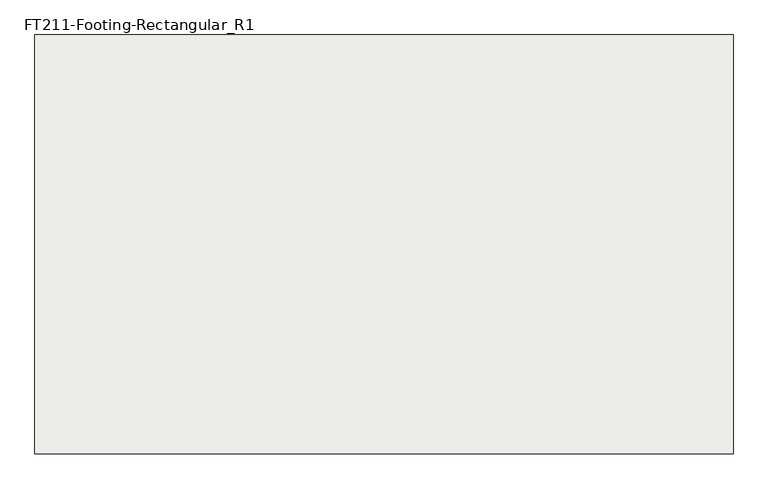
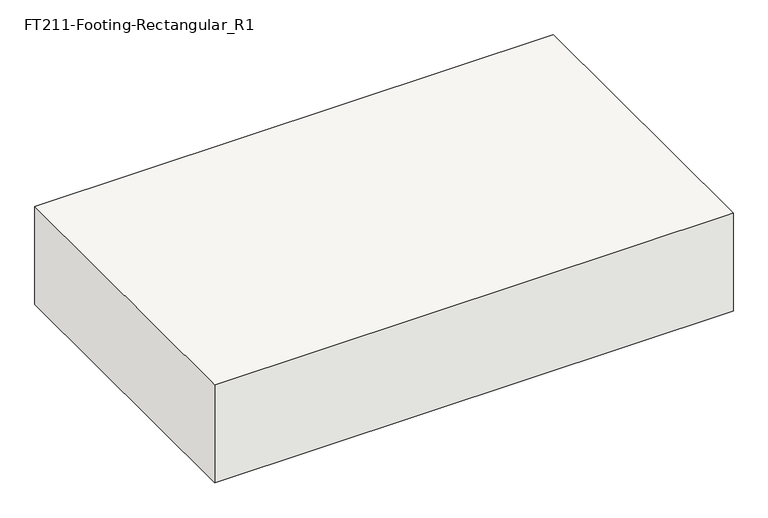
"""IFC4 building model written with IfcOpenShell, lengths in millimetres: slab geometry, FT211-Footing-Rectangular_R1 : H_SF_ACF_W2500xL1500xT500_Bitumen."""

import ifcopenshell
import ifcopenshell.guid

model = None  # the IFC model being written
_history = None  # IfcOwnerHistory: only IFC2X3 demands one
_inside = {}  # id of a spatial element -> (the spatial element, [elements in it])
_under = {}  # id of a project, library or spatial element -> (it, [spatial elements below it])
_declared = {}  # id of a project -> (the project, [libraries it declares])
_typed = {}  # id of a type object -> (the type object, [elements of that type])
_made_of = {}  # id of a material, layer set ... -> (it, [elements and type objects made of it])


def new_model(schema):
    """Start an empty IFC model of exactly this schema.

    Asked for "IFC4X3", IfcOpenShell would pick the latest addendum, in which some entities
    have other attributes; the version numbers below select the first issue.
    IFC2X3 requires an IfcOwnerHistory on every rooted entity: one is made here for all.
    """
    global model, _history
    if schema == "IFC4X3":
        model = ifcopenshell.file(schema_version=(4, 3, 0, 0))
    else:
        model = ifcopenshell.file(schema=schema)
    _inside.clear()
    _under.clear()
    _declared.clear()
    _typed.clear()
    _made_of.clear()
    _history = None
    if model.schema == "IFC2X3":
        org = make("IfcOrganization", Name="unknown")
        user = make(
            "IfcPersonAndOrganization",
            ThePerson=make("IfcPerson", FamilyName="unknown"),
            TheOrganization=org,
        )
        app = make(
            "IfcApplication",
            ApplicationDeveloper=org,
            Version="unknown",
            ApplicationFullName="unknown",
            ApplicationIdentifier="unknown",
        )
        _history = make(
            "IfcOwnerHistory",
            OwningUser=user,
            OwningApplication=app,
            ChangeAction="ADDED",
            CreationDate=0,
        )
    return model


def make(cls, **values):
    """One entity of the class cls with the attributes given. An attribute that is None is left unset."""
    return model.create_entity(
        cls, **{name: value for name, value in values.items() if value is not None}
    )


def rooted(cls, **values):
    """An entity with a GlobalId (a new one), such as an element, a storey or a relation."""
    return make(cls, GlobalId=ifcopenshell.guid.new(), OwnerHistory=_history, **values)


def si_unit(unit_type, name, prefix=None):
    """IfcSIUnit, for example si_unit("LENGTHUNIT", "METRE", prefix="MILLI")."""
    return make("IfcSIUnit", UnitType=unit_type, Prefix=prefix, Name=name)


def assignment(units):
    """IfcUnitAssignment: the units of a project."""
    return None if units is None else make("IfcUnitAssignment", Units=units)


def point(xyz):
    """IfcCartesianPoint."""
    return None if xyz is None else make("IfcCartesianPoint", Coordinates=xyz)


def direction(xyz):
    """IfcDirection."""
    return None if xyz is None else make("IfcDirection", DirectionRatios=xyz)


def frame(location, z_axis=None, x_axis=None):
    """IfcAxis2Placement3D, a coordinate frame: its origin and axes. An axis left out is left unset."""
    return make(
        "IfcAxis2Placement3D",
        Location=point(location),
        Axis=direction(z_axis),
        RefDirection=direction(x_axis),
    )


def origin():
    """The frame at (0, 0, 0) with its axes left unset."""
    return frame((0.0, 0.0, 0.0))


def place(relative_to, where):
    """IfcLocalPlacement: puts the frame where relative to a parent placement (None: the world)."""
    return make(
        "IfcLocalPlacement", PlacementRelTo=relative_to, RelativePlacement=where
    )


def context(
    kind, dimensions, precision=None, world=None, true_north=None, identifier=None
):
    """IfcGeometricRepresentationContext, for example the 3D "Model" context."""
    return make(
        "IfcGeometricRepresentationContext",
        ContextIdentifier=identifier,
        ContextType=kind,
        CoordinateSpaceDimension=dimensions,
        Precision=precision,
        WorldCoordinateSystem=world,
        TrueNorth=true_north,
    )


def project(units=None, contexts=None):
    """IfcProject with its units and contexts."""
    return rooted(
        "IfcProject",
        Name="project",
        RepresentationContexts=contexts,
        UnitsInContext=assignment(units),
    )


def spatial(cls, under=None, at=None, **own):
    """A site, building, storey or space (cls), placed at a placement, below another one or the project."""
    s = rooted(cls, ObjectPlacement=at, **own)
    if under is not None:
        _under.setdefault(under.id(), (under, []))[1].append(s)
    return s


def polyline(points):
    """IfcPolyline through the points."""
    return make("IfcPolyline", Points=[point(p) for p in points])


def outline(outer, holes=None, kind="AREA"):
    """IfcArbitraryClosedProfileDef: a profile drawn as a closed curve; with holes, ...WithVoids."""
    if holes is None:
        return make("IfcArbitraryClosedProfileDef", ProfileType=kind, OuterCurve=outer)
    return make(
        "IfcArbitraryProfileDefWithVoids",
        ProfileType=kind,
        OuterCurve=outer,
        InnerCurves=holes,
    )


def extrude(swept, where, along, depth):
    """IfcExtrudedAreaSolid: the profile swept, set in the frame where, extruded along a direction by depth."""
    return make(
        "IfcExtrudedAreaSolid",
        SweptArea=swept,
        Position=where,
        ExtrudedDirection=direction(along),
        Depth=depth,
    )


def shape(context_of_items, identifier, shape_type, items):
    """IfcShapeRepresentation: the items that make up one representation, for example the "Body"."""
    return make(
        "IfcShapeRepresentation",
        ContextOfItems=context_of_items,
        RepresentationIdentifier=identifier,
        RepresentationType=shape_type,
        Items=items,
    )


def source(mapping_origin, context_of_items, identifier, shape_type, items):
    """IfcRepresentationMap: a shape defined once, which mapped items show again and again."""
    return make(
        "IfcRepresentationMap",
        MappingOrigin=mapping_origin,
        MappedRepresentation=shape(context_of_items, identifier, shape_type, items),
    )


def transform(
    local_origin,
    x_axis=None,
    y_axis=None,
    z_axis=None,
    scale=None,
    scale2=None,
    scale3=None,
    uniform=True,
):
    """IfcCartesianTransformationOperator3D, or its non-uniform kind. x_axis, y_axis, z_axis: its Axis1, 2, 3."""
    if uniform:
        return make(
            "IfcCartesianTransformationOperator3D",
            Axis1=direction(x_axis),
            Axis2=direction(y_axis),
            LocalOrigin=point(local_origin),
            Scale=scale,
            Axis3=direction(z_axis),
        )
    return make(
        "IfcCartesianTransformationOperator3DnonUniform",
        Axis1=direction(x_axis),
        Axis2=direction(y_axis),
        LocalOrigin=point(local_origin),
        Scale=scale,
        Axis3=direction(z_axis),
        Scale2=scale2,
        Scale3=scale3,
    )


def mapped(mapping_source, mapping_target):
    """IfcMappedItem: shows the shape of a source again, moved by a transform."""
    return make(
        "IfcMappedItem", MappingSource=mapping_source, MappingTarget=mapping_target
    )


def made_of(thing, what):
    """Note that an element or type object is made of a material, layer set ...; save() writes the relation."""
    if what is not None:
        _made_of.setdefault(what.id(), (what, []))[1].append(thing)
    return thing


def element(
    cls,
    number,
    at=None,
    inside=None,
    cuts=None,
    type_object=None,
    material=None,
    context=None,
    identifier="Body",
    shape_type=None,
    held_by="IfcProductDefinitionShape",
    body=None,
    shapes=None,
    **own,
):
    """One element of the class cls, such as IfcWall. Its Tag is "e" and its number.

    at: its placement. inside: the storey or other place that contains it. cuts: it is an
    opening in that element (IfcRelVoidsElement). A single representation is given by context,
    identifier, shape_type and body (its items); several are given by shapes. held_by: the class
    of the entity that holds the representations. save() writes the other relations.
    """
    e = rooted(cls, Tag="e%d" % number, ObjectPlacement=at, **own)
    if body is not None:
        shapes = [shape(context, identifier, shape_type, body)]
    if shapes is not None:
        e.Representation = make(held_by, Representations=shapes)
    if inside is not None:
        _inside.setdefault(inside.id(), (inside, []))[1].append(e)
    if cuts is not None:
        rooted(
            "IfcRelVoidsElement", RelatingBuildingElement=cuts, RelatedOpeningElement=e
        )
    if type_object is not None:
        _typed.setdefault(type_object.id(), (type_object, []))[1].append(e)
    return made_of(e, material)


def aggregate(whole, parts):
    """IfcRelAggregates: a whole, such as a stair, and the parts it consists of."""
    return rooted("IfcRelAggregates", RelatingObject=whole, RelatedObjects=parts)


def save(model, path):
    """Write the relations noted so far, then the file.

    IfcRelAggregates (storeys below a building ...), IfcRelContainedInSpatialStructure (elements
    in a storey), IfcRelDefinesByType, IfcRelAssociatesMaterial and IfcRelDeclares: one each for
    every whole, place, type object, material and project.
    """
    for whole, parts in _under.values():
        aggregate(whole, parts)
    for where, things in _inside.values():
        rooted(
            "IfcRelContainedInSpatialStructure",
            RelatedElements=things,
            RelatingStructure=where,
        )
    for kind, things in _typed.values():
        rooted("IfcRelDefinesByType", RelatedObjects=things, RelatingType=kind)
    for what, things in _made_of.values():
        rooted("IfcRelAssociatesMaterial", RelatedObjects=things, RelatingMaterial=what)
    for by, libraries in _declared.values():
        rooted("IfcRelDeclares", RelatingContext=by, RelatedDefinitions=libraries)
    model.write(path)


def ft211_footing_rectangular_r1_907a7f09(model_context):
    return source(origin(), model_context, "Body", "SweptSolid", [
        extrude(outline(polyline([(1250.0, 750.0), (1250.0, -750.0), (-1250.0, -750.0), (-1250.0, 750.0), (1250.0, 750.0)])), frame((0.0, 0.0, -500.0), z_axis=(0.0, 0.0, 1.0), x_axis=(1.0, 0.0, 0.0)), (0.0, 0.0, 1.0), 500.0),
    ])


if __name__ == "__main__":
    model = new_model("IFC4")
    model_context = context("Model", 3, world=origin())
    ifc_project = project(units=[si_unit("LENGTHUNIT", "METRE", prefix="MILLI")], contexts=[model_context])
    site = spatial("IfcSite", under=ifc_project)
    building = spatial("IfcBuilding", under=site)
    placement = place(None, origin())
    ft211_footing_rectangular_r1_shape = ft211_footing_rectangular_r1_907a7f09(model_context)
    element("IfcSlab", 1, ObjectType="FT211-Footing-Rectangular_R1 : H_SF_ACF_W2500xL1500xT500_Bitumen", at=placement, inside=building, context=model_context, shape_type="MappedRepresentation", body=[
        mapped(ft211_footing_rectangular_r1_shape, transform((0.0, 0.0, 0.0), x_axis=(1.0, 0.0, 0.0), y_axis=(0.0, 1.0, 0.0), z_axis=(0.0, 0.0, 1.0))),
    ])
    save(model, "model.ifc")

# Revit data of these elements
# Type "FT211-Footing-Rectangular_R1 : H_SF_ACF_W2500xL1500xT500_Bitumen"
#   Top bar = "D25@300"
#   Description = "UG Shallow Foundation"
#   Bottom bar = "D20@300"
#   Width = 2500.000 mm
#   Length = 1500.000 mm
#   Foundation Thickness = 500.000 mm
#   Structural Material [instance default] = none
#   Assembly Code = ""
